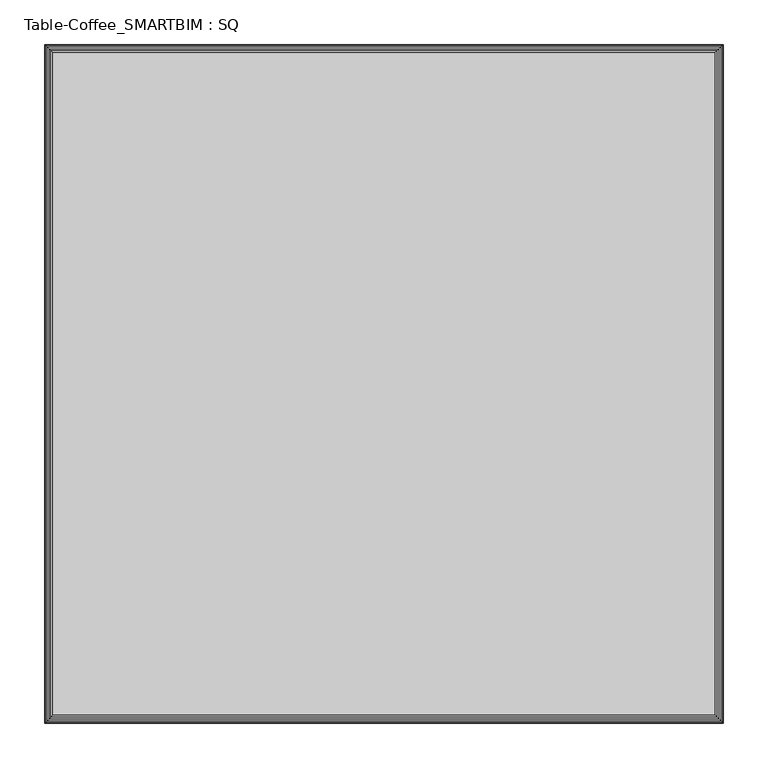
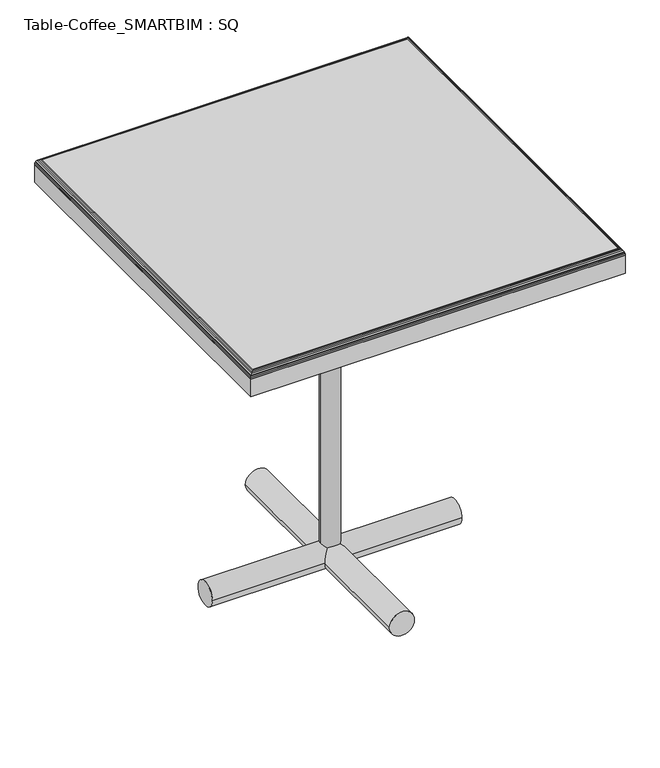
"""IFC4 building model written with IfcOpenShell, lengths in millimetres: furniture geometry, Table-Coffee_SMARTBIM : SQ."""

import ifcopenshell
import ifcopenshell.guid

model = None  # the IFC model being written
_history = None  # IfcOwnerHistory: only IFC2X3 demands one
_inside = {}  # id of a spatial element -> (the spatial element, [elements in it])
_under = {}  # id of a project, library or spatial element -> (it, [spatial elements below it])
_declared = {}  # id of a project -> (the project, [libraries it declares])
_typed = {}  # id of a type object -> (the type object, [elements of that type])
_made_of = {}  # id of a material, layer set ... -> (it, [elements and type objects made of it])


def new_model(schema):
    """Start an empty IFC model of exactly this schema.

    Asked for "IFC4X3", IfcOpenShell would pick the latest addendum, in which some entities
    have other attributes; the version numbers below select the first issue.
    IFC2X3 requires an IfcOwnerHistory on every rooted entity: one is made here for all.
    """
    global model, _history
    if schema == "IFC4X3":
        model = ifcopenshell.file(schema_version=(4, 3, 0, 0))
    else:
        model = ifcopenshell.file(schema=schema)
    _inside.clear()
    _under.clear()
    _declared.clear()
    _typed.clear()
    _made_of.clear()
    _history = None
    if model.schema == "IFC2X3":
        org = make("IfcOrganization", Name="unknown")
        user = make(
            "IfcPersonAndOrganization",
            ThePerson=make("IfcPerson", FamilyName="unknown"),
            TheOrganization=org,
        )
        app = make(
            "IfcApplication",
            ApplicationDeveloper=org,
            Version="unknown",
            ApplicationFullName="unknown",
            ApplicationIdentifier="unknown",
        )
        _history = make(
            "IfcOwnerHistory",
            OwningUser=user,
            OwningApplication=app,
            ChangeAction="ADDED",
            CreationDate=0,
        )
    return model


def make(cls, **values):
    """One entity of the class cls with the attributes given. An attribute that is None is left unset."""
    return model.create_entity(
        cls, **{name: value for name, value in values.items() if value is not None}
    )


def rooted(cls, **values):
    """An entity with a GlobalId (a new one), such as an element, a storey or a relation."""
    return make(cls, GlobalId=ifcopenshell.guid.new(), OwnerHistory=_history, **values)


def si_unit(unit_type, name, prefix=None):
    """IfcSIUnit, for example si_unit("LENGTHUNIT", "METRE", prefix="MILLI")."""
    return make("IfcSIUnit", UnitType=unit_type, Prefix=prefix, Name=name)


def assignment(units):
    """IfcUnitAssignment: the units of a project."""
    return None if units is None else make("IfcUnitAssignment", Units=units)


def point(xyz):
    """IfcCartesianPoint."""
    return None if xyz is None else make("IfcCartesianPoint", Coordinates=xyz)


def direction(xyz):
    """IfcDirection."""
    return None if xyz is None else make("IfcDirection", DirectionRatios=xyz)


def frame(location, z_axis=None, x_axis=None):
    """IfcAxis2Placement3D, a coordinate frame: its origin and axes. An axis left out is left unset."""
    return make(
        "IfcAxis2Placement3D",
        Location=point(location),
        Axis=direction(z_axis),
        RefDirection=direction(x_axis),
    )


def frame_2d(location, x_axis=None):
    """IfcAxis2Placement2D, a coordinate frame in the plane: its origin and x axis."""
    return make(
        "IfcAxis2Placement2D", Location=point(location), RefDirection=direction(x_axis)
    )


def origin():
    """The frame at (0, 0, 0) with its axes left unset."""
    return frame((0.0, 0.0, 0.0))


def origin_2d():
    """The frame at (0, 0) in the plane with its x axis left unset."""
    return frame_2d((0.0, 0.0))


def place(relative_to, where):
    """IfcLocalPlacement: puts the frame where relative to a parent placement (None: the world)."""
    return make(
        "IfcLocalPlacement", PlacementRelTo=relative_to, RelativePlacement=where
    )


def context(
    kind, dimensions, precision=None, world=None, true_north=None, identifier=None
):
    """IfcGeometricRepresentationContext, for example the 3D "Model" context."""
    return make(
        "IfcGeometricRepresentationContext",
        ContextIdentifier=identifier,
        ContextType=kind,
        CoordinateSpaceDimension=dimensions,
        Precision=precision,
        WorldCoordinateSystem=world,
        TrueNorth=true_north,
    )


def project(units=None, contexts=None):
    """IfcProject with its units and contexts."""
    return rooted(
        "IfcProject",
        Name="project",
        RepresentationContexts=contexts,
        UnitsInContext=assignment(units),
    )


def spatial(cls, under=None, at=None, **own):
    """A site, building, storey or space (cls), placed at a placement, below another one or the project."""
    s = rooted(cls, ObjectPlacement=at, **own)
    if under is not None:
        _under.setdefault(under.id(), (under, []))[1].append(s)
    return s


def polyline(points):
    """IfcPolyline through the points."""
    return make("IfcPolyline", Points=[point(p) for p in points])


def circle_curve(where, radius):
    """IfcCircle in the frame where."""
    return make("IfcCircle", Position=where, Radius=radius)


def ellipse_curve(where, semi_axis1, semi_axis2):
    """IfcEllipse in the frame where."""
    return make(
        "IfcEllipse", Position=where, SemiAxis1=semi_axis1, SemiAxis2=semi_axis2
    )


def trimmed(basis, trim1, trim2, sense, master):
    """IfcTrimmedCurve: the piece of a basis curve between two trims."""
    return make(
        "IfcTrimmedCurve",
        BasisCurve=basis,
        Trim1=trim1,
        Trim2=trim2,
        SenseAgreement=sense,
        MasterRepresentation=master,
    )


def segment(curve, same_sense, transition):
    """IfcCompositeCurveSegment."""
    return make(
        "IfcCompositeCurveSegment",
        Transition=transition,
        SameSense=same_sense,
        ParentCurve=curve,
    )


def composite_curve(segments, self_intersect=None):
    """IfcCompositeCurve: segments joined end to end."""
    return make("IfcCompositeCurve", Segments=segments, SelfIntersect=self_intersect)


def outline(outer, holes=None, kind="AREA"):
    """IfcArbitraryClosedProfileDef: a profile drawn as a closed curve; with holes, ...WithVoids."""
    if holes is None:
        return make("IfcArbitraryClosedProfileDef", ProfileType=kind, OuterCurve=outer)
    return make(
        "IfcArbitraryProfileDefWithVoids",
        ProfileType=kind,
        OuterCurve=outer,
        InnerCurves=holes,
    )


def extrude(swept, where, along, depth):
    """IfcExtrudedAreaSolid: the profile swept, set in the frame where, extruded along a direction by depth."""
    return make(
        "IfcExtrudedAreaSolid",
        SweptArea=swept,
        Position=where,
        ExtrudedDirection=direction(along),
        Depth=depth,
    )


def shape(context_of_items, identifier, shape_type, items):
    """IfcShapeRepresentation: the items that make up one representation, for example the "Body"."""
    return make(
        "IfcShapeRepresentation",
        ContextOfItems=context_of_items,
        RepresentationIdentifier=identifier,
        RepresentationType=shape_type,
        Items=items,
    )


def source(mapping_origin, context_of_items, identifier, shape_type, items):
    """IfcRepresentationMap: a shape defined once, which mapped items show again and again."""
    return make(
        "IfcRepresentationMap",
        MappingOrigin=mapping_origin,
        MappedRepresentation=shape(context_of_items, identifier, shape_type, items),
    )


def transform(
    local_origin,
    x_axis=None,
    y_axis=None,
    z_axis=None,
    scale=None,
    scale2=None,
    scale3=None,
    uniform=True,
):
    """IfcCartesianTransformationOperator3D, or its non-uniform kind. x_axis, y_axis, z_axis: its Axis1, 2, 3."""
    if uniform:
        return make(
            "IfcCartesianTransformationOperator3D",
            Axis1=direction(x_axis),
            Axis2=direction(y_axis),
            LocalOrigin=point(local_origin),
            Scale=scale,
            Axis3=direction(z_axis),
        )
    return make(
        "IfcCartesianTransformationOperator3DnonUniform",
        Axis1=direction(x_axis),
        Axis2=direction(y_axis),
        LocalOrigin=point(local_origin),
        Scale=scale,
        Axis3=direction(z_axis),
        Scale2=scale2,
        Scale3=scale3,
    )


def mapped(mapping_source, mapping_target):
    """IfcMappedItem: shows the shape of a source again, moved by a transform."""
    return make(
        "IfcMappedItem", MappingSource=mapping_source, MappingTarget=mapping_target
    )


def made_of(thing, what):
    """Note that an element or type object is made of a material, layer set ...; save() writes the relation."""
    if what is not None:
        _made_of.setdefault(what.id(), (what, []))[1].append(thing)
    return thing


def element(
    cls,
    number,
    at=None,
    inside=None,
    cuts=None,
    type_object=None,
    material=None,
    context=None,
    identifier="Body",
    shape_type=None,
    held_by="IfcProductDefinitionShape",
    body=None,
    shapes=None,
    **own,
):
    """One element of the class cls, such as IfcWall. Its Tag is "e" and its number.

    at: its placement. inside: the storey or other place that contains it. cuts: it is an
    opening in that element (IfcRelVoidsElement). A single representation is given by context,
    identifier, shape_type and body (its items); several are given by shapes. held_by: the class
    of the entity that holds the representations. save() writes the other relations.
    """
    e = rooted(cls, Tag="e%d" % number, ObjectPlacement=at, **own)
    if body is not None:
        shapes = [shape(context, identifier, shape_type, body)]
    if shapes is not None:
        e.Representation = make(held_by, Representations=shapes)
    if inside is not None:
        _inside.setdefault(inside.id(), (inside, []))[1].append(e)
    if cuts is not None:
        rooted(
            "IfcRelVoidsElement", RelatingBuildingElement=cuts, RelatedOpeningElement=e
        )
    if type_object is not None:
        _typed.setdefault(type_object.id(), (type_object, []))[1].append(e)
    return made_of(e, material)


def aggregate(whole, parts):
    """IfcRelAggregates: a whole, such as a stair, and the parts it consists of."""
    return rooted("IfcRelAggregates", RelatingObject=whole, RelatedObjects=parts)


def save(model, path):
    """Write the relations noted so far, then the file.

    IfcRelAggregates (storeys below a building ...), IfcRelContainedInSpatialStructure (elements
    in a storey), IfcRelDefinesByType, IfcRelAssociatesMaterial and IfcRelDeclares: one each for
    every whole, place, type object, material and project.
    """
    for whole, parts in _under.values():
        aggregate(whole, parts)
    for where, things in _inside.values():
        rooted(
            "IfcRelContainedInSpatialStructure",
            RelatedElements=things,
            RelatingStructure=where,
        )
    for kind, things in _typed.values():
        rooted("IfcRelDefinesByType", RelatedObjects=things, RelatingType=kind)
    for what, things in _made_of.values():
        rooted("IfcRelAssociatesMaterial", RelatedObjects=things, RelatingMaterial=what)
    for by, libraries in _declared.values():
        rooted("IfcRelDeclares", RelatingContext=by, RelatedDefinitions=libraries)
    model.write(path)


def plane_surface(at):
    """IfcPlane: the flat surface through the origin of the frame at, square to its z axis."""
    return make("IfcPlane", Position=at)


def cylinder_surface(at, radius):
    """IfcCylindricalSurface: all points at the distance radius from the z axis of the frame at."""
    return make("IfcCylindricalSurface", Position=at, Radius=radius)


def advanced_brep(points, edges, surfaces, faces):
    """IfcAdvancedBrep: a solid bounded by faces that lie on surfaces and meet in shared edges.

    An edge is (start, end): straight between two places in points (the first is 0);
    or (start, end, curve); or (start, end, curve, False) where it runs against its curve.
    A face is (place in surfaces, loops), or (place, loops, False) where it looks against
    its surface's normal. A loop lists edges by number (the first is 1), with a minus sign
    where the edge is run from its end to its start. The first loop is the outer one.
    """
    corners = [point(p) for p in points]
    vertices = [make("IfcVertexPoint", VertexGeometry=c) for c in corners]
    made = []
    for start, end, *more in edges:
        made.append(
            make(
                "IfcEdgeCurve",
                EdgeStart=vertices[start],
                EdgeEnd=vertices[end],
                EdgeGeometry=more[0] if more else make("IfcPolyline", Points=[corners[start], corners[end]]),
                SameSense=more[1] if len(more) > 1 else True,
            )
        )
    hull = []
    for where, loops, *sense in faces:
        bounds = []
        for j, loop in enumerate(loops):
            ring = [make("IfcOrientedEdge", EdgeElement=made[abs(k) - 1], Orientation=k > 0) for k in loop]
            bounds.append(
                make(
                    "IfcFaceOuterBound" if j == 0 else "IfcFaceBound",
                    Bound=make("IfcEdgeLoop", EdgeList=ring),
                    Orientation=True,
                )
            )
        hull.append(make("IfcAdvancedFace", Bounds=bounds, FaceSurface=surfaces[where], SameSense=sense[0] if sense else True))
    return make("IfcAdvancedBrep", Outer=make("IfcClosedShell", CfsFaces=hull))


def table_coffee_smartbim_sq_4378fec3(model_context):
    return source(origin(), model_context, "Body", "SolidModel", [
        extrude(outline(composite_curve([segment(trimmed(circle_curve(frame_2d((0.0, 25.4)), 25.4), [point((25.4, 25.4))], [point((-25.4, 25.4))], False, "CARTESIAN"), True, "CONTINUOUS"), segment(trimmed(circle_curve(frame_2d((0.0, 25.4)), 25.4), [point((-25.4, 25.4))], [point((25.4, 25.4))], False, "CARTESIAN"), True, "CONTINUOUS")], self_intersect=False)), frame((-254.0, 0.0, 0.0), z_axis=(1.0, 0.0, 0.0), x_axis=(0.0, 1.0, 0.0)), (0.0, 0.0, 1.0), 508.0),
        extrude(outline(composite_curve([segment(trimmed(circle_curve(frame_2d((25.4, 0.0)), 25.4), [point((25.4, -25.4))], [point((25.4, 25.4))], False, "CARTESIAN"), True, "CONTINUOUS"), segment(trimmed(circle_curve(frame_2d((25.4, 0.0)), 25.4), [point((25.4, 25.4))], [point((25.4, -25.4))], False, "CARTESIAN"), True, "CONTINUOUS")], self_intersect=False)), frame((0.0, -254.0, 0.0), z_axis=(0.0, 1.0, 0.0), x_axis=(0.0, 0.0, 1.0)), (0.0, 0.0, 1.0), 508.0),
        extrude(outline(polyline([(381.0, 381.0), (381.0, -381.0), (-381.0, -381.0), (-381.0, 381.0), (381.0, 381.0)])), frame((0.0, 0.0, 723.9), z_axis=(0.0, 0.0, 1.0), x_axis=(1.0, 0.0, 0.0)), (0.0, 0.0, 1.0), 38.1),
        advanced_brep(
        [(-371.5998654, -371.5998654, 774.7), (371.5998654, -371.5998654, 774.7), (371.5998654, 371.5998654, 774.7), (-371.5998654, 371.5998654, 774.7), (381.0, 381.0, 762.0), (381.0, -381.0, 762.0), (-381.0, -381.0, 762.0), (-381.0, 381.0, 762.0), (-381.0, 381.0, 765.2998654), (381.0, 381.0, 765.2998654), (-381.0, -381.0, 765.2998654), (381.0, -381.0, 765.2998654), (-380.6372483, -380.6372483, 767.8860287), (-380.6372483, 380.6372483, 767.8860287), (-373.7616212, 373.7616212, 774.4480533), (-373.7616212, -373.7616212, 774.4480533), (-375.7639185, 375.7639185, 773.7273912), (-375.7639185, -375.7639185, 773.7273912), (-377.8885738, 377.8885738, 772.2866155), (-377.8885738, -377.8885738, 772.2866155), (-379.9102962, 379.9102962, 769.692959), (-379.9102962, -379.9102962, 769.692959), (380.6372483, -380.6372483, 767.8860287), (373.7616212, -373.7616212, 774.4480533), (375.7639185, -375.7639185, 773.7273912), (377.8885738, -377.8885738, 772.2866155), (379.9102962, -379.9102962, 769.692959), (380.6372483, 380.6372483, 767.8860287), (373.7616212, 373.7616212, 774.4480533), (375.7639185, 375.7639185, 773.7273912), (377.8885738, 377.8885738, 772.2866155), (379.9102962, 379.9102962, 769.692959)],
        [
            (0, 1),
            (1, 2),
            (2, 3),
            (3, 0),
            (4, 5),
            (5, 6),
            (6, 7),
            (7, 4),
            (7, 8),
            (8, 9),
            (9, 4),
            (6, 10),
            (10, 8),
            (5, 11),
            (11, 10),
            (9, 11),
            (10, 12, ellipse_curve(frame((-371.5998654, -371.5998654, 765.2998654), z_axis=(-0.7071067811865475, 0.7071067811865475, 0.0), x_axis=(-0.7071067811865474, -0.7071067811865476, 0.0)), 13.2937978, 9.4001346)),
            (12, 13),
            (13, 8, ellipse_curve(frame((-371.5998654, 371.5998654, 765.2998654), z_axis=(-0.7071067811865475, -0.7071067811865475, 0.0), x_axis=(0.7071067811865474, -0.7071067811865476, 0.0)), 13.2937978, 9.4001346)),
            (14, 15),
            (15, 0, ellipse_curve(frame((-371.5998654, -371.5998654, 765.2998654), z_axis=(-0.7071067811865475, 0.7071067811865475, 0.0), x_axis=(-0.7071067811865474, -0.7071067811865476, 0.0)), 13.2937978, 9.4001346)),
            (3, 14, ellipse_curve(frame((-371.5998654, 371.5998654, 765.2998654), z_axis=(-0.7071067811865475, -0.7071067811865475, 0.0), x_axis=(0.7071067811865474, -0.7071067811865476, 0.0)), 13.2937978, 9.4001346)),
            (14, 16, ellipse_curve(frame((-371.5998654, 371.5998654, 765.2998654), z_axis=(-0.7071067811865475, -0.7071067811865475, 0.0), x_axis=(0.7071067811865474, -0.7071067811865476, 0.0)), 13.2937978, 9.4001346)),
            (16, 17),
            (17, 15, ellipse_curve(frame((-371.5998654, -371.5998654, 765.2998654), z_axis=(-0.7071067811865475, 0.7071067811865475, 0.0), x_axis=(-0.7071067811865474, -0.7071067811865476, 0.0)), 13.2937978, 9.4001346)),
            (16, 18, ellipse_curve(frame((-371.5998654, 371.5998654, 765.2998654), z_axis=(-0.7071067811865475, -0.7071067811865475, 0.0), x_axis=(0.7071067811865474, -0.7071067811865476, 0.0)), 13.2937978, 9.4001346)),
            (18, 19),
            (19, 17, ellipse_curve(frame((-371.5998654, -371.5998654, 765.2998654), z_axis=(-0.7071067811865475, 0.7071067811865475, 0.0), x_axis=(-0.7071067811865474, -0.7071067811865476, 0.0)), 13.2937978, 9.4001346)),
            (18, 20, ellipse_curve(frame((-371.5998654, 371.5998654, 765.2998654), z_axis=(-0.7071067811865475, -0.7071067811865475, 0.0), x_axis=(0.7071067811865474, -0.7071067811865476, 0.0)), 13.2937978, 9.4001346)),
            (20, 21),
            (21, 19, ellipse_curve(frame((-371.5998654, -371.5998654, 765.2998654), z_axis=(-0.7071067811865475, 0.7071067811865475, 0.0), x_axis=(-0.7071067811865474, -0.7071067811865476, 0.0)), 13.2937978, 9.4001346)),
            (12, 21, ellipse_curve(frame((-371.5998654, -371.5998654, 765.2998654), z_axis=(-0.7071067811865475, 0.7071067811865475, 0.0), x_axis=(-0.7071067811865474, -0.7071067811865476, 0.0)), 13.2937978, 9.4001346)),
            (20, 13, ellipse_curve(frame((-371.5998654, 371.5998654, 765.2998654), z_axis=(-0.7071067811865475, -0.7071067811865475, 0.0), x_axis=(0.7071067811865474, -0.7071067811865476, 0.0)), 13.2937978, 9.4001346)),
            (11, 22, ellipse_curve(frame((371.5998654, -371.5998654, 765.2998654), z_axis=(-0.7071067811865475, -0.7071067811865475, 0.0), x_axis=(0.7071067811865476, -0.7071067811865474, 0.0)), 13.2937978, 9.4001346)),
            (22, 12),
            (15, 23),
            (23, 1, ellipse_curve(frame((371.5998654, -371.5998654, 765.2998654), z_axis=(-0.7071067811865475, -0.7071067811865475, 0.0), x_axis=(0.7071067811865476, -0.7071067811865474, 0.0)), 13.2937978, 9.4001346)),
            (17, 24),
            (24, 23, ellipse_curve(frame((371.5998654, -371.5998654, 765.2998654), z_axis=(-0.7071067811865475, -0.7071067811865475, 0.0), x_axis=(0.7071067811865476, -0.7071067811865474, 0.0)), 13.2937978, 9.4001346)),
            (19, 25),
            (25, 24, ellipse_curve(frame((371.5998654, -371.5998654, 765.2998654), z_axis=(-0.7071067811865475, -0.7071067811865475, 0.0), x_axis=(0.7071067811865476, -0.7071067811865474, 0.0)), 13.2937978, 9.4001346)),
            (21, 26),
            (26, 25, ellipse_curve(frame((371.5998654, -371.5998654, 765.2998654), z_axis=(-0.7071067811865475, -0.7071067811865475, 0.0), x_axis=(0.7071067811865476, -0.7071067811865474, 0.0)), 13.2937978, 9.4001346)),
            (22, 26, ellipse_curve(frame((371.5998654, -371.5998654, 765.2998654), z_axis=(-0.7071067811865475, -0.7071067811865475, 0.0), x_axis=(0.7071067811865476, -0.7071067811865474, 0.0)), 13.2937978, 9.4001346)),
            (9, 27, ellipse_curve(frame((371.5998654, 371.5998654, 765.2998654), z_axis=(0.7071067811865475, -0.7071067811865475, 0.0), x_axis=(0.7071067811865474, 0.7071067811865476, 0.0)), 13.2937978, 9.4001346)),
            (27, 22),
            (23, 28),
            (28, 2, ellipse_curve(frame((371.5998654, 371.5998654, 765.2998654), z_axis=(0.7071067811865475, -0.7071067811865475, 0.0), x_axis=(0.7071067811865474, 0.7071067811865476, 0.0)), 13.2937978, 9.4001346)),
            (24, 29),
            (29, 28, ellipse_curve(frame((371.5998654, 371.5998654, 765.2998654), z_axis=(0.7071067811865475, -0.7071067811865475, 0.0), x_axis=(0.7071067811865474, 0.7071067811865476, 0.0)), 13.2937978, 9.4001346)),
            (25, 30),
            (30, 29, ellipse_curve(frame((371.5998654, 371.5998654, 765.2998654), z_axis=(0.7071067811865475, -0.7071067811865475, 0.0), x_axis=(0.7071067811865474, 0.7071067811865476, 0.0)), 13.2937978, 9.4001346)),
            (26, 31),
            (31, 30, ellipse_curve(frame((371.5998654, 371.5998654, 765.2998654), z_axis=(0.7071067811865475, -0.7071067811865475, 0.0), x_axis=(0.7071067811865474, 0.7071067811865476, 0.0)), 13.2937978, 9.4001346)),
            (27, 31, ellipse_curve(frame((371.5998654, 371.5998654, 765.2998654), z_axis=(0.7071067811865475, -0.7071067811865475, 0.0), x_axis=(0.7071067811865474, 0.7071067811865476, 0.0)), 13.2937978, 9.4001346)),
            (13, 27),
            (28, 14),
            (29, 16),
            (30, 18),
            (31, 20),
        ],
        [
            plane_surface(frame((-381.0, 381.0, 774.7), z_axis=(0.0, 0.0, 1.0), x_axis=(-1.0, 0.0, 0.0))),
            plane_surface(frame((-381.0, 381.0, 762.0), z_axis=(0.0, 0.0, -1.0), x_axis=(1.0, 0.0, 0.0))),
            plane_surface(frame((381.0, 381.0, 774.7), z_axis=(0.0, 1.0, 0.0), x_axis=(0.0, 0.0, -1.0))),
            plane_surface(frame((-381.0, 381.0, 774.7), z_axis=(-1.0, 0.0, 0.0), x_axis=(0.0, 0.0, -1.0))),
            plane_surface(frame((-381.0, -381.0, 774.7), z_axis=(0.0, -1.0, 0.0), x_axis=(0.0, 0.0, -1.0))),
            plane_surface(frame((381.0, -381.0, 774.7), z_axis=(1.0, 0.0, 0.0), x_axis=(0.0, 0.0, -1.0))),
            cylinder_surface(frame((-371.5998654, 381.0, 765.2998654), z_axis=(0.0, -1.0, 0.0), x_axis=(1.0, 0.0, 0.0)), 9.4001346),
            cylinder_surface(frame((-381.0, -371.5998654, 765.2998654), z_axis=(1.0, 0.0, 0.0), x_axis=(0.0, 1.0, 0.0)), 9.4001346),
            cylinder_surface(frame((371.5998654, -381.0, 765.2998654), z_axis=(0.0, 1.0, 0.0), x_axis=(-1.0, 0.0, 0.0)), 9.4001346),
            cylinder_surface(frame((381.0, 371.5998654, 765.2998654), z_axis=(-1.0, 0.0, 0.0), x_axis=(0.0, -1.0, 0.0)), 9.4001346),
        ],
        [
            (0, [[1, 2, 3, 4]]),
            (1, [[5, 6, 7, 8]]),
            (2, [[-8, 9, 10, 11]]),
            (3, [[-7, 12, 13, -9]]),
            (4, [[-6, 14, 15, -12]]),
            (5, [[-5, -11, 16, -14]]),
            (6, [[17, 18, 19, -13]]),
            (6, [[20, 21, -4, 22]]),
            (6, [[-20, 23, 24, 25]]),
            (6, [[-24, 26, 27, 28]]),
            (6, [[-27, 29, 30, 31]]),
            (6, [[-18, 32, -30, 33]]),
            (7, [[-17, -15, 34, 35]]),
            (7, [[-21, 36, 37, -1]]),
            (7, [[-25, 38, 39, -36]]),
            (7, [[-28, 40, 41, -38]]),
            (7, [[-31, 42, 43, -40]]),
            (7, [[-32, -35, 44, -42]]),
            (8, [[-34, -16, 45, 46]]),
            (8, [[-37, 47, 48, -2]]),
            (8, [[-39, 49, 50, -47]]),
            (8, [[-41, 51, 52, -49]]),
            (8, [[-43, 53, 54, -51]]),
            (8, [[-44, -46, 55, -53]]),
            (9, [[-19, 56, -45, -10]]),
            (9, [[-22, -3, -48, 57]]),
            (9, [[-23, -57, -50, 58]]),
            (9, [[-26, -58, -52, 59]]),
            (9, [[-29, -59, -54, 60]]),
            (9, [[-33, -60, -55, -56]]),
        ],
    ),
        extrude(outline(polyline([(76.2, 76.2), (76.2, -76.2), (-76.2, -76.2), (-76.2, 76.2), (76.2, 76.2)])), frame((0.0, 0.0, 755.65), z_axis=(0.0, 0.0, 1.0), x_axis=(1.0, 0.0, 0.0)), (0.0, 0.0, 1.0), 6.35),
        extrude(outline(composite_curve([segment(trimmed(circle_curve(origin_2d(), 19.05), [point((-19.05, 0.0))], [point((19.05, 0.0))], False, "CARTESIAN"), True, "CONTINUOUS"), segment(trimmed(circle_curve(origin_2d(), 19.05), [point((19.05, 0.0))], [point((-19.05, 0.0))], False, "CARTESIAN"), True, "CONTINUOUS")], self_intersect=False)), frame((0.0, 0.0, 24.2070278), z_axis=(0.0, 0.0, 1.0), x_axis=(1.0, 0.0, 0.0)), (0.0, 0.0, 1.0), 731.4429722),
    ])


if __name__ == "__main__":
    model = new_model("IFC4")
    model_context = context("Model", 3, world=origin())
    ifc_project = project(units=[si_unit("LENGTHUNIT", "METRE", prefix="MILLI")], contexts=[model_context])
    site = spatial("IfcSite", under=ifc_project)
    building = spatial("IfcBuilding", under=site)
    placement = place(None, origin())
    table_coffee_smartbim_sq_shape = table_coffee_smartbim_sq_4378fec3(model_context)
    element("IfcFurniture", 1, ObjectType="Table-Coffee_SMARTBIM : SQ", at=placement, inside=building, context=model_context, shape_type="MappedRepresentation", body=[
        mapped(table_coffee_smartbim_sq_shape, transform((0.0, 0.0, 0.0), x_axis=(1.0, 0.0, 0.0), y_axis=(0.0, 1.0, 0.0), z_axis=(0.0, 0.0, 1.0))),
    ])
    save(model, "model.ifc")

# Revit data of these elements
# Type "Table-Coffee_SMARTBIM : SQ"
#   Subcategory = "Table\r\n"
#   SmartBIM Object Created By = "SMARTBIM, LLC"
#   Manufacturer = "SMARTBIM"
#   Assembly Code = "E2020200"
#   95 CSI = "12500"
#   04 CSI = "12 50 00"
#   table cloth = 0' - 1 1/2"
#   Width = 2' - 6"
#   SmartBIM Object Version = 3
#   Height = 2' - 6"
#   Depth = 2' - 6"
#   Default Elevation = 4' - 0"
#   white cloth_parameter = WOOD-OAKFIRE
#   Table Unit = MET
#   Glide = none
#   Glass = none
# Element 1 (IfcFurniture, "Table-Coffee_SMARTBIM : SQ")
#   Materials on its faces: "WOOD-OAKFIRE", "MET"
# Materials
#   "WOOD-OAKFIRE": class "Wood", colour RGB 198 202 183, transparency 0, Description = "Generic wood", Cost = 0
#   "MET": class "Metal", colour RGB 189 187 185, transparency 0
